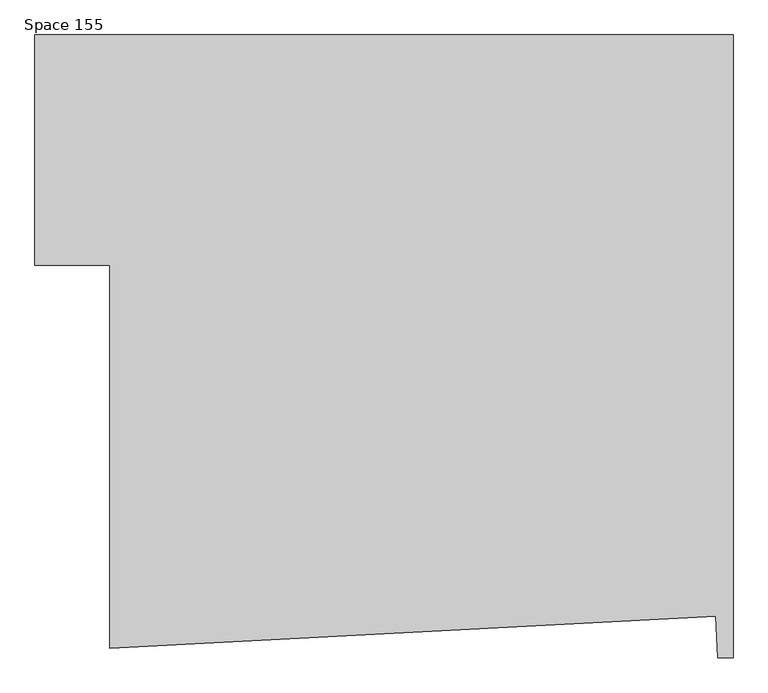
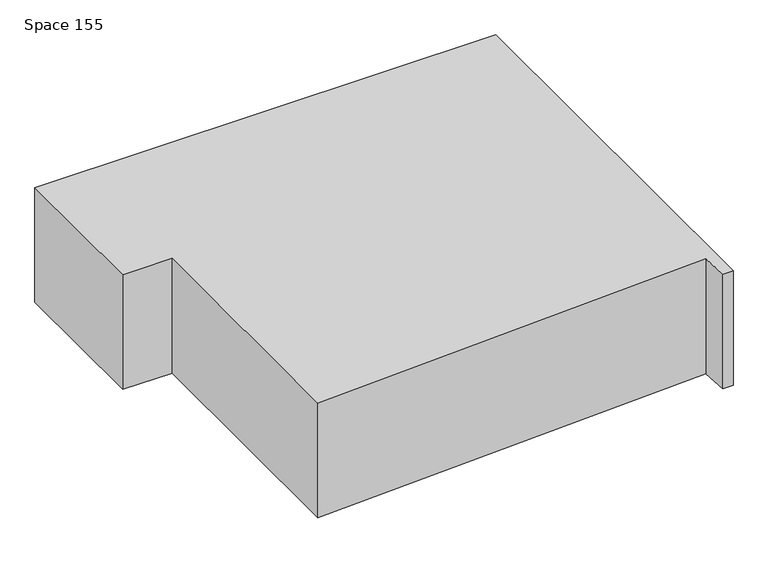
"""IFC4 building model written with IfcOpenShell, lengths in millimetres: proxy geometry, Space 155."""

from ifc_helpers import new_model, si_unit, frame, origin, place, context, project, spatial, polyline, outline, extrude, source, transform, mapped, element, save


def space_155_4a308f5e(model_context):
    return source(origin(), model_context, "Body", "SweptSolid", [
        extrude(outline(polyline([(22947.3559655, 11513.340365), (21705.9309655, 11513.340365), (21705.9309655, 15336.040365), (33291.5059655, 15336.040365), (33291.5059655, 4998.240365), (33037.5425464, 4998.240365), (33001.5254261, 5685.4879602), (22947.3559655, 5158.5712663), (22947.3559655, 11513.340365)])), frame((0.0, 0.0, 3810.0), z_axis=(0.0, 0.0, 1.0), x_axis=(1.0, 0.0, 0.0)), (0.0, 0.0, 1.0), 3048.0),
    ])


if __name__ == "__main__":
    model = new_model("IFC4")
    model_context = context("Model", 3, world=origin())
    ifc_project = project(units=[si_unit("LENGTHUNIT", "METRE", prefix="MILLI")], contexts=[model_context])
    site = spatial("IfcSite", under=ifc_project)
    building = spatial("IfcBuilding", under=site)
    placement = place(None, origin())
    space_155_shape = space_155_4a308f5e(model_context)
    element("IfcBuildingElementProxy", 1, Name="Space 155", ObjectType="Space 155", at=placement, inside=building, context=model_context, shape_type="MappedRepresentation", body=[
        mapped(space_155_shape, transform((0.0, 0.0, 0.0), x_axis=(1.0, 0.0, 0.0), y_axis=(0.0, 1.0, 0.0), z_axis=(0.0, 0.0, 1.0))),
    ])
    save(model, "model.ifc")

# Revit data of these elements
# Element 1 (IfcBuildingElementProxy, "Space 155")
#   Materials on its faces: "Render Material 255-255-255"
# Materials
#   "Render Material 255-255-255": class "Unassigned", colour RGB 255 255 255, transparency 0
